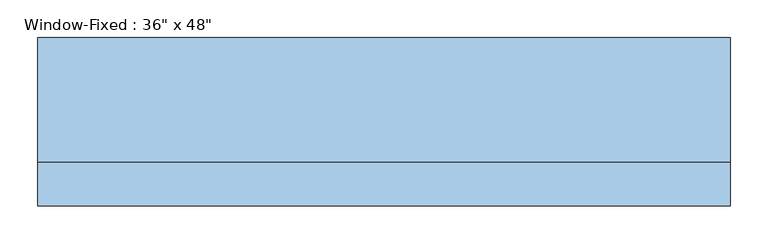
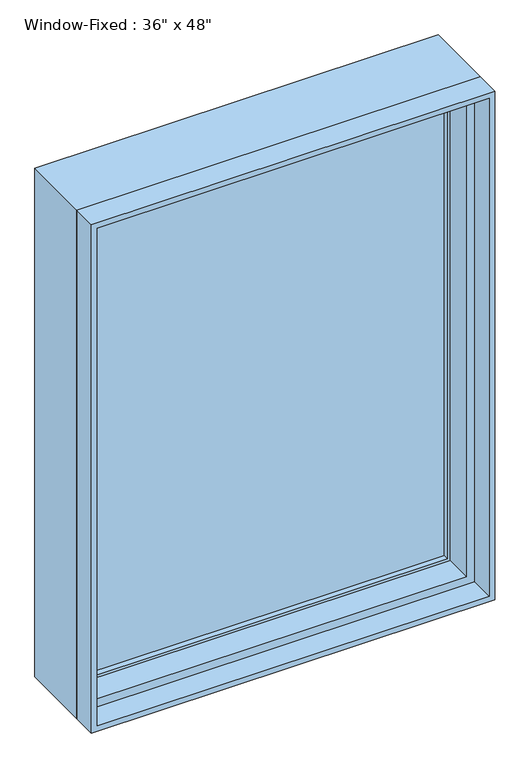
"""IFC4 building model written with IfcOpenShell, lengths in millimetres: window geometry."""

from ifc_helpers import new_model, si_unit, frame, origin, place, context, project, spatial, polyline, outline, extrude, faceted_brep, source, transform, mapped, element, save


def window_0c0f7d0c(model_context):
    return source(origin(), model_context, "Body", "SolidModel", [
        extrude(outline(polyline([(419.1, 50.6984), (419.1, 44.3484), (-419.1, 44.3484), (-419.1, 50.6984), (419.1, 50.6984)])), frame((0.0, 0.0, 952.5), z_axis=(0.0, 0.0, 1.0), x_axis=(1.0, 0.0, 0.0)), (0.0, 0.0, 1.0), 1143.0),
        extrude(outline(polyline([(-419.1, 31.6484), (-419.1, 37.9984), (419.1, 37.9984), (419.1, 31.6484), (-419.1, 31.6484)])), frame((0.0, 0.0, 952.5), z_axis=(0.0, 0.0, 1.0), x_axis=(1.0, 0.0, 0.0)), (0.0, 0.0, 1.0), 1143.0),
        extrude(outline(polyline([(927.1, 444.5), (2120.9, 444.5), (2120.9, -444.5), (927.1, -444.5), (927.1, 444.5)]), holes=[polyline([(952.5, -419.1), (2095.5, -419.1), (2095.5, 419.1), (952.5, 419.1), (952.5, -419.1)])]), frame((0.0, 18.9484, 0.0), z_axis=(0.0, 1.0, 0.0), x_axis=(0.0, 0.0, 1.0)), (0.0, 0.0, 1.0), 44.45),
        extrude(outline(polyline([(2133.6, -457.2), (914.4, -457.2), (914.4, 457.2), (2133.6, 457.2), (2133.6, -457.2)]), holes=[polyline([(2120.9, 444.5), (927.1, 444.5), (927.1, -444.5), (2120.9, -444.5), (2120.9, 444.5)])]), frame((0.0, -101.6, 0.0), z_axis=(0.0, 1.0, 0.0), x_axis=(0.0, 0.0, 1.0)), (0.0, 0.0, 1.0), 57.0484),
        faceted_brep([(457.2, -44.5516, 2133.6), (457.2, 120.65, 2133.6), (-457.2, 120.65, 2133.6), (-457.2, -44.5516, 2133.6), (-457.2, 120.65, 914.4), (-457.2, -44.5516, 914.4), (457.2, 120.65, 914.4), (457.2, -44.5516, 914.4), (425.45, -44.5516, 2101.85), (425.45, -44.5516, 946.15), (-425.45, -44.5516, 946.15), (-425.45, -44.5516, 2101.85), (-444.5, 120.65, 2120.9), (-444.5, 120.65, 927.1), (444.5, 120.65, 927.1), (444.5, 120.65, 2120.9), (425.45, 18.9484, 2101.85), (-425.45, 18.9484, 2101.85), (444.5, 18.9484, 2120.9), (-444.5, 18.9484, 2120.9), (-425.45, 18.9484, 946.15), (-444.5, 18.9484, 927.1), (425.45, 18.9484, 946.15), (444.5, 18.9484, 927.1)], [[[0, 1, 2, 3]], [[3, 2, 4, 5]], [[5, 4, 6, 7]], [[3, 5, 7, 0], [8, 9, 10, 11]], [[7, 6, 1, 0]], [[1, 6, 4, 2], [12, 13, 14, 15]], [[16, 8, 11, 17]], [[15, 18, 19, 12]], [[17, 11, 10, 20]], [[12, 19, 21, 13]], [[20, 10, 9, 22]], [[13, 21, 23, 14]], [[22, 9, 8, 16]], [[18, 23, 21, 19], [17, 20, 22, 16]], [[14, 23, 18, 15]]]),
    ])


if __name__ == "__main__":
    model = new_model("IFC4")
    model_context = context("Model", 3, world=origin())
    ifc_project = project(units=[si_unit("LENGTHUNIT", "METRE", prefix="MILLI")], contexts=[model_context])
    site = spatial("IfcSite", under=ifc_project)
    building = spatial("IfcBuilding", under=site)
    placement = place(None, origin())
    window_shape = window_0c0f7d0c(model_context)
    element("IfcWindow", 1, ObjectType="Window-Fixed : 36\" x 48\"", at=placement, inside=building, context=model_context, shape_type="MappedRepresentation", body=[
        mapped(window_shape, transform((0.0, 0.0, 0.0), x_axis=(1.0, 0.0, 0.0), y_axis=(0.0, 1.0, 0.0), z_axis=(0.0, 0.0, 1.0))),
    ])
    save(model, "model.ifc")

# Revit data of these elements
# Type "Window-Fixed : 36\" x 48\""
#   Type Mark = "1"
#   Fire Rating = "0.5h"
#   Assembly Code = "B2020100"
#   Analytic Construction = "Double glazing - domestic"
#   Window Inset [instance default] = 0.00 ft
#   Wall Thickness [instance default] = 0.50 ft
#   Visual Light Transmittance = 0.81
#   Thermal Resistance (R) = 1.8146 (h·ft²·°F)/BTU
#   Solar Heat Gain Coefficient = 0.76
#   Rough Width = 3.041667 ft
#   Rough Height = 4.041667 ft
#   Interior Wall Closure [instance default] = 0.1875 ft
#   Height = 4.00 ft
#   Heat Transfer Coefficient (U) = 0.5511 BTU/(h·ft²·°F)
#   Frame Extension [instance default] = 0.020833 ft
#   Exterior Wall Closure [instance default] = 0.104167 ft
#   Extension Jamb [instance default] = 0.1875 ft
#   Default Sill Height = 3.00 ft
#   Width = 3.00 ft
#   Muntin Visibility = yes
#   Interior Trim Visibility [instance default] = yes
#   Exterior Trim Visibility [instance default] = yes
#   Extension Jamb Visibility [instance default] = yes
#   Muntin Pattern = Muntin Pattern_2x2 : Muntin Pattern_2x2
#   Interior Trim Material = Maple - Semigloss
#   Interior Trim = Trim-Window-Interior-Flat : Picture Frame
#   Interior Frame Material = Maple - Semigloss
#   Glass Panel Material = Glass, Clear Glazing
#   Exterior Trim Material = Clad - White
#   Exterior Trim = Trim-Window-Exterior-Flat : with Sill
#   Exterior Frame Material = Clad - White
#   Wall Closure = (empty or 0)
# Element 1 (IfcWindow, "Window-Fixed : 36\" x 48\"")
#   Window Inset = 0.167 ft
#   Wall Thickness = 0.666667 ft
#   Frame Extension = 0.187833 ft
#   Extension Jamb = 0.187167 ft
#   Materials on its faces: "Maple - Semigloss", "Glass, Clear Glazing", "Clad - White"
# Materials
#   "Maple - Semigloss": class "Wood", colour RGB 196 161 118, transparency 0, Description = "Acer Saccharum", Cost = 0
#   "Glass, Clear Glazing": class "Glass", colour RGB 245 245 243, transparency 1, Description = "Clear glazing", Cost = 0
#   "Clad - White": class "Wood", colour RGB 245 245 243, transparency 0, Cost = 0
